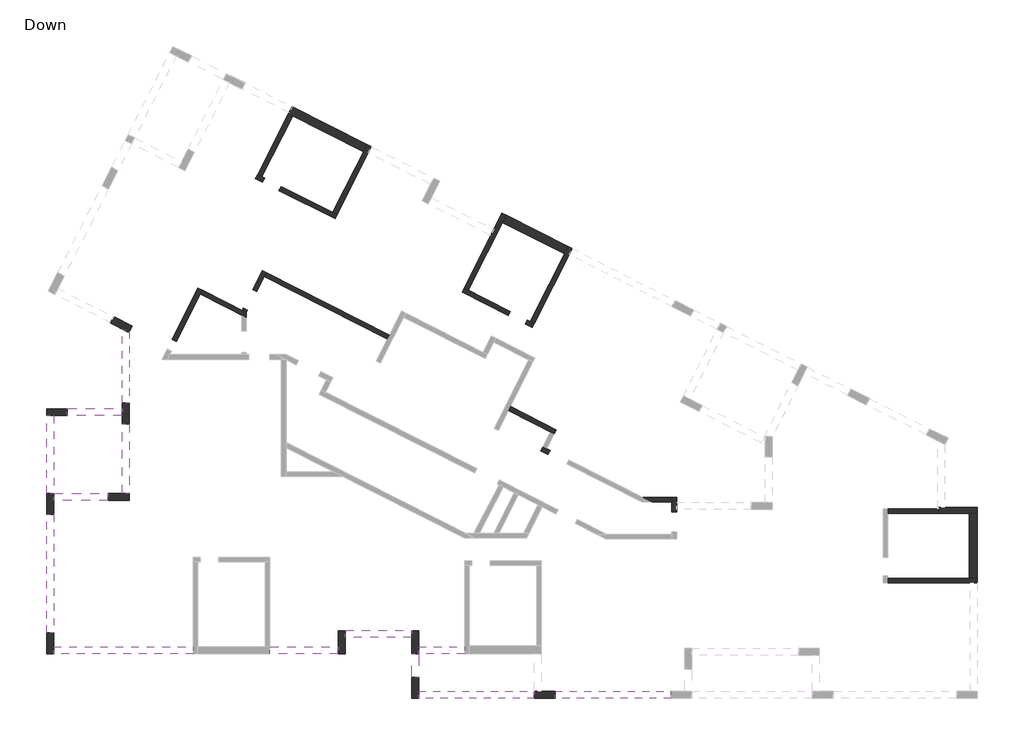
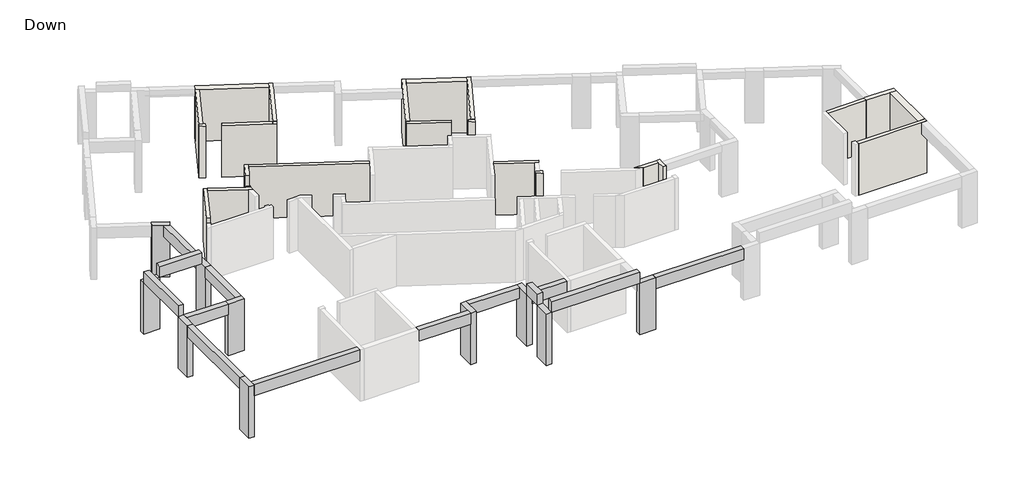
# One storey, part 2 of 3: 23 walls, 13 beams, 10 columns.
"""IFC4 building model written with IfcOpenShell, lengths in millimetres."""

from ifc_helpers import new_model, si_unit, frame, origin, origin_with_axes, place, context, project, spatial, polyline, outline, extrude, faceted_brep, element, save

model = new_model("IFC4")

# Units and contexts
model_context = context("Model", 3, world=origin())
ifc_project = project(units=[si_unit("LENGTHUNIT", "METRE", prefix="MILLI")], contexts=[model_context])

# Site, building, storey
site = spatial("IfcSite", under=ifc_project)
building = spatial("IfcBuilding", under=site)
storey = spatial("IfcBuildingStorey", under=building, Name="Down", Elevation=0.0)

# Beams
placement = place(None, origin())
element("IfcBeam", 1, ObjectType="Concrete Rectengular Beam : 30/65", at=placement, inside=storey, context=model_context, shape_type="SweptSolid", body=[
    extrude(outline(polyline([(-20357.3945771, -8406.9823068), (-20057.3945771, -8406.9823068), (-20057.3945771, -13520.1864188), (-20357.3945771, -13520.1864188), (-20357.3945771, -8406.9823068)])), frame((0.0, 0.0, 2430.0), z_axis=(0.0, 0.0, 1.0), x_axis=(1.0, 0.0, 0.0)), (0.0, 0.0, 1.0), 650.0),
])
element("IfcBeam", 2, ObjectType="Concrete Rectengular Beam : 30/65", at=placement, inside=storey, context=model_context, shape_type="Brep", body=[
    faceted_brep([(-17693.6398388, -7806.9823068, 3080.0), (-17693.6398388, -7506.9823068, 3080.0), (-20057.3945771, -7506.9823068, 3080.0), (-20057.3945771, -7806.9823068, 3080.0), (-20057.3945771, -7806.9823068, 2780.0), (-20057.3945771, -7806.9823068, 2430.0), (-17693.6398388, -7806.9823068, 2430.0), (-17693.6398388, -7806.9823068, 2780.0), (-17693.6398388, -7506.9823068, 2430.0), (-20057.3945771, -7506.9823068, 2430.0)], [[[0, 1, 2, 3]], [[0, 3, 4, 5, 6, 7]], [[8, 6, 5, 9]], [[1, 8, 9, 2]], [[1, 0, 7, 6, 8]], [[3, 2, 9, 5, 4]]]),
])
element("IfcBeam", 3, ObjectType="Concrete Rectengular Beam : 30/65", at=placement, inside=storey, context=model_context, shape_type="Brep", body=[
    faceted_brep([(-16793.6398388, -4507.7754014, 3080.0), (-17093.6398388, -4507.7754014, 3080.0), (-17093.6398388, -7506.9823068, 3080.0), (-16793.6398388, -7506.9823068, 3080.0), (-16793.6398388, -7506.9823068, 2780.0), (-16793.6398388, -7506.9823068, 2430.0), (-16793.6398388, -4507.7754014, 2430.0), (-16793.6398388, -4507.7754014, 2780.0), (-17093.6398388, -4507.7754014, 2430.0), (-17093.6398388, -7506.9823068, 2430.0)], [[[0, 1, 2, 3]], [[0, 3, 4, 5, 6, 7]], [[8, 6, 5, 9]], [[1, 8, 9, 2]], [[1, 0, 7, 6, 8]], [[3, 2, 9, 5, 4]]]),
])
element("IfcBeam", 4, ObjectType="Concrete Rectengular Beam : 30/65", at=placement, inside=storey, context=model_context, shape_type="Brep", body=[
    faceted_brep([(-17093.6398388, -3607.7754014, 3080.0), (-16793.6398388, -3607.7754014, 3080.0), (-16793.6398388, -532.9875537, 3080.0), (-16809.6695875, -564.4305223, 3080.0), (-17093.6398388, -419.6613746, 3080.0), (-16793.6398388, -3607.7754014, 2780.0), (-16793.6398388, -3607.7754014, 2430.0), (-16793.6398388, -532.9875537, 2430.0), (-16793.6398388, -532.9875537, 2780.0), (-17093.6398388, -3607.7754014, 2430.0), (-17093.6398388, -419.6613746, 2430.0), (-16809.6695875, -564.4305223, 2430.0)], [[[0, 1, 2, 3, 4]], [[2, 1, 5, 6, 7, 8]], [[6, 9, 10, 11, 7]], [[4, 10, 9, 0]], [[1, 0, 9, 6, 5]], [[3, 11, 10, 4]], [[11, 3, 2, 8, 7]]]),
])
element("IfcBeam", 5, ObjectType="Concrete Rectengular Beam : 30/65", at=placement, inside=storey, context=model_context, shape_type="Brep", body=[
    faceted_brep([(-20057.3945771, -14116.2328988, 3080.0), (-20057.3945771, -14416.2328988, 3080.0), (-14040.0148736, -14416.2328988, 3080.0), (-14040.0148736, -14116.2328988, 3080.0), (-20057.3945771, -14116.2328988, 2430.0), (-20057.3945771, -14116.2328988, 2780.0), (-14040.0148736, -14116.2328988, 2780.0), (-14040.0148736, -14116.2328988, 2430.0), (-20057.3945771, -14416.2328988, 2430.0), (-14040.0148736, -14416.2328988, 2430.0)], [[[0, 1, 2, 3]], [[4, 5, 0, 3, 6, 7]], [[8, 4, 7, 9]], [[1, 8, 9, 2]], [[1, 0, 5, 4, 8]], [[3, 2, 9, 7, 6]]]),
])
element("IfcBeam", 6, ObjectType="Concrete Rectengular Beam : 30/65", at=placement, inside=storey, context=model_context, shape_type="Brep", body=[
    faceted_brep([(-7799.9037617, -14416.2328988, 3080.0), (-7799.9037617, -14116.2328988, 3080.0), (-10738.2112055, -14116.2328988, 3080.0), (-10738.2112055, -14416.2328988, 3080.0), (-7799.9037617, -14416.2328988, 2430.0), (-10738.2112055, -14416.2328988, 2430.0), (-7799.9037617, -14116.2328988, 2430.0), (-10738.2112055, -14116.2328988, 2430.0), (-7799.9037617, -14116.2328988, 2780.0), (-10738.2112055, -14116.2328988, 2780.0)], [[[0, 1, 2, 3]], [[4, 0, 3, 5]], [[6, 4, 5, 7]], [[1, 8, 6, 7, 9, 2]], [[1, 0, 4, 6, 8]], [[3, 2, 9, 7, 5]]]),
])
element("IfcBeam", 7, ObjectType="Concrete Rectengular Beam : 30/65", at=placement, inside=storey, context=model_context, shape_type="Brep", body=[
    faceted_brep([(-7499.9037617, -13416.2328988, 3080.0), (-7499.9037617, -13716.2328988, 3080.0), (-4637.2823123, -13716.2328988, 3080.0), (-4637.2823123, -13416.2328988, 3080.0), (-7499.9037617, -13716.2328988, 2430.0), (-4637.2823123, -13716.2328988, 2430.0), (-7499.9037617, -13416.2328988, 2430.0), (-4637.2823123, -13416.2328988, 2430.0), (-4637.2823123, -13416.2328988, 2780.0), (-7499.9037617, -13416.2328988, 2780.0)], [[[0, 1, 2, 3]], [[1, 4, 5, 2]], [[4, 6, 7, 5]], [[0, 3, 8, 7, 6, 9]], [[1, 0, 9, 6, 4]], [[3, 2, 5, 7, 8]]]),
])
element("IfcBeam", 8, ObjectType="Concrete Rectengular Beam : 30/65", at=placement, inside=storey, context=model_context, shape_type="Brep", body=[
    faceted_brep([(-4337.2823123, -14116.2328988, 3080.0), (-4337.2823123, -14416.2328988, 3080.0), (-2356.7095864, -14416.2328988, 3080.0), (-2356.7095864, -14116.2328988, 3080.0), (-4337.2823123, -14416.2328988, 2430.0), (-2356.7095864, -14416.2328988, 2430.0), (-4337.2823123, -14116.2328988, 2430.0), (-2356.7095864, -14116.2328988, 2430.0), (-4337.2823123, -14116.2328988, 2780.0), (-2356.7095864, -14116.2328988, 2780.0)], [[[0, 1, 2, 3]], [[1, 4, 5, 2]], [[4, 6, 7, 5]], [[6, 8, 0, 3, 9, 7]], [[1, 0, 8, 6, 4]], [[3, 2, 5, 7, 9]]]),
])
element("IfcBeam", 9, ObjectType="Concrete Rectengular Beam : 30/65", at=placement, inside=storey, context=model_context, shape_type="SweptSolid", body=[
    extrude(outline(polyline([(1545.0940817, -16335.9823018), (1545.0940817, -16035.9823018), (6525.6343679, -16035.9823018), (6525.6343679, -16335.9823018), (1545.0940817, -16335.9823018)])), frame((0.0, 0.0, 2430.0), z_axis=(0.0, 0.0, 1.0), x_axis=(1.0, 0.0, 0.0)), (0.0, 0.0, 1.0), 650.0),
])
element("IfcBeam", 10, ObjectType="Concrete Rectengular Beam : 30/65", at=placement, inside=storey, context=model_context, shape_type="SweptSolid", body=[
    extrude(outline(polyline([(-20059.1333783, -7506.9823068), (-20359.1333783, -7506.9823068), (-20359.1333783, -4157.1728829), (-20059.1333783, -4157.1728829), (-20059.1333783, -7506.9823068)])), frame((0.0, 0.0, 3080.0), z_axis=(0.0, 0.0, 1.0), x_axis=(1.0, 0.0, 0.0)), (0.0, 0.0, 1.0), 650.0),
])
element("IfcBeam", 11, ObjectType="Concrete Rectengular Beam : 30/65", at=placement, inside=storey, context=model_context, shape_type="SweptSolid", body=[
    extrude(outline(polyline([(-17093.6398388, -3857.1728829), (-17093.6398388, -4157.1728829), (-19459.1333783, -4157.1728829), (-19459.1333783, -3857.1728829), (-17093.6398388, -3857.1728829)])), frame((0.0, 0.0, 3080.0), z_axis=(0.0, 0.0, 1.0), x_axis=(1.0, 0.0, 0.0)), (0.0, 0.0, 1.0), 650.0),
])
element("IfcBeam", 12, ObjectType="Concrete Rectengular Beam : 30/65", at=placement, inside=storey, context=model_context, shape_type="SweptSolid", body=[
    extrude(outline(polyline([(-4337.2823123, -15437.5523212), (-4637.2823123, -15437.5523212), (-4637.2823123, -14416.2328988), (-4337.2823123, -14416.2328988), (-4337.2823123, -15437.5523212)])), frame((0.0, 0.0, 3080.0), z_axis=(0.0, 0.0, 1.0), x_axis=(1.0, 0.0, 0.0)), (0.0, 0.0, 1.0), 650.0),
])
element("IfcBeam", 13, ObjectType="Concrete Rectengular Beam : 30/65", at=placement, inside=storey, context=model_context, shape_type="SweptSolid", body=[
    extrude(outline(polyline([(645.0940817, -16035.9823018), (645.0940817, -16335.9823018), (-4337.2823123, -16335.9823018), (-4337.2823123, -16035.9823018), (645.0940817, -16035.9823018)])), frame((0.0, 0.0, 3080.0), z_axis=(0.0, 0.0, 1.0), x_axis=(1.0, 0.0, 0.0)), (0.0, 0.0, 1.0), 650.0),
])

# Columns
element("IfcColumn", 14, ObjectType="Concrete Rectengular Column : 30/100", at=placement, inside=storey, context=model_context, shape_type="Brep", body=[
    faceted_brep([(-7499.9037617, -13416.2328988, 0.0), (-7499.9037617, -14416.2328988, 0.0), (-7799.9037617, -14416.2328988, 0.0), (-7799.9037617, -13416.2328988, 0.0), (-7499.9037617, -13416.2328988, 3080.0), (-7499.9037617, -14416.2328988, 3080.0), (-7799.9037617, -14416.2328988, 3080.0), (-7799.9037617, -14116.2328988, 3080.0), (-7799.9037617, -13416.2328988, 3080.0), (-7799.9037617, -13416.2328988, 2780.0)], [[[0, 1, 2, 3]], [[4, 5, 1, 0]], [[5, 6, 2, 1]], [[6, 7, 8, 9, 3, 2]], [[8, 4, 0, 3, 9]], [[4, 8, 7, 6, 5]]]),
])
element("IfcColumn", 15, ObjectType="Concrete Rectengular Column : 30/100", at=placement, inside=storey, context=model_context, shape_type="Brep", body=[
    faceted_brep([(-4337.2823123, -13416.2328988, 0.0), (-4337.2823123, -14416.2328988, 0.0), (-4637.2823123, -14416.2328988, 0.0), (-4637.2823123, -13416.2328988, 0.0), (-4337.2823123, -13416.2328988, 3080.0), (-4337.2823123, -14116.2328988, 3080.0), (-4337.2823123, -14416.2328988, 3080.0), (-4337.2823123, -13416.2328988, 2780.0), (-4637.2823123, -14416.2328988, 3080.0), (-4637.2823123, -13416.2328988, 3080.0)], [[[0, 1, 2, 3]], [[4, 5, 6, 1, 0, 7]], [[6, 8, 2, 1]], [[8, 9, 3, 2]], [[9, 4, 7, 0, 3]], [[4, 9, 8, 6, 5]]]),
])
element("IfcColumn", 16, ObjectType="Concrete Rectengular Column : 30/90", at=placement, inside=storey, context=model_context, shape_type="SweptSolid", body=[
    extrude(outline(polyline([(-20359.1333783, -3857.1728829), (-19459.1333783, -3857.1728829), (-19459.1333783, -4157.1728829), (-20359.1333783, -4157.1728829), (-20359.1333783, -3857.1728829)])), origin_with_axes(), (0.0, 0.0, 1.0), 3080.0),
])
element("IfcColumn", 17, ObjectType="Concrete Rectengular Column : 30/90", at=placement, inside=storey, context=model_context, shape_type="SweptSolid", body=[
    extrude(outline(polyline([(-17093.6398388, -4507.7754014), (-17093.6398388, -3607.7754014), (-16793.6398388, -3607.7754014), (-16793.6398388, -4507.7754014), (-17093.6398388, -4507.7754014)])), origin_with_axes(), (0.0, 0.0, 1.0), 3080.0),
])
element("IfcColumn", 18, ObjectType="Concrete Rectengular Column : 30/90", at=placement, inside=storey, context=model_context, shape_type="Brep", body=[
    faceted_brep([(-20357.3945771, -8406.9823068, 0.0), (-20357.3945771, -7506.9823068, 0.0), (-20057.3945771, -7506.9823068, 0.0), (-20057.3945771, -8406.9823068, 0.0), (-20357.3945771, -8406.9823068, 3080.0), (-20357.3945771, -7506.9823068, 3080.0), (-20057.3945771, -7506.9823068, 3080.0), (-20057.3945771, -7806.9823068, 3080.0), (-20057.3945771, -8406.9823068, 3080.0)], [[[0, 1, 2, 3]], [[4, 5, 1, 0]], [[5, 6, 2, 1]], [[6, 7, 8, 3, 2]], [[8, 4, 0, 3]], [[4, 8, 7, 6, 5]]]),
])
element("IfcColumn", 19, ObjectType="Concrete Rectengular Column : 30/90", at=placement, inside=storey, context=model_context, shape_type="Brep", body=[
    faceted_brep([(-16793.6398388, -7806.9823068, 0.0), (-17693.6398388, -7806.9823068, 0.0), (-17693.6398388, -7506.9823068, 0.0), (-16793.6398388, -7506.9823068, 0.0), (-16793.6398388, -7806.9823068, 3080.0), (-17693.6398388, -7806.9823068, 3080.0), (-16793.6398388, -7806.9823068, 2780.0), (-17693.6398388, -7506.9823068, 3080.0), (-16793.6398388, -7506.9823068, 3080.0)], [[[0, 1, 2, 3]], [[4, 5, 1, 0, 6]], [[5, 7, 2, 1]], [[7, 8, 3, 2]], [[8, 4, 6, 0, 3]], [[4, 8, 7, 5]]]),
])
element("IfcColumn", 20, ObjectType="Concrete Rectengular Column : 30/90", at=placement, inside=storey, context=model_context, shape_type="Brep", body=[
    faceted_brep([(-20057.3945771, -13520.1864188, 0.0), (-20057.3945771, -14420.1864188, 0.0), (-20357.3945771, -14420.1864188, 0.0), (-20357.3945771, -13520.1864188, 0.0), (-20057.3945771, -13520.1864188, 3080.0), (-20057.3945771, -14116.2328988, 3080.0), (-20057.3945771, -14420.1864188, 3080.0), (-20357.3945771, -14420.1864188, 3080.0), (-20357.3945771, -13520.1864188, 3080.0)], [[[0, 1, 2, 3]], [[4, 5, 6, 1, 0]], [[6, 7, 2, 1]], [[7, 8, 3, 2]], [[8, 4, 0, 3]], [[4, 8, 7, 6, 5]]]),
])
element("IfcColumn", 21, ObjectType="Concrete Rectengular Column : 30/90", at=placement, inside=storey, context=model_context, shape_type="SweptSolid", body=[
    extrude(outline(polyline([(-4337.2823123, -15437.5523212), (-4337.2823123, -16337.5523212), (-4637.2823123, -16337.5523212), (-4637.2823123, -15437.5523212), (-4337.2823123, -15437.5523212)])), origin_with_axes(), (0.0, 0.0, 1.0), 3080.0),
])
element("IfcColumn", 22, ObjectType="Concrete Rectengular Column : 30/90", at=placement, inside=storey, context=model_context, shape_type="Brep", body=[
    faceted_brep([(645.0940817, -16035.9823018, 0.0), (1545.0940817, -16035.9823018, 0.0), (1545.0940817, -16335.9823018, 0.0), (645.0940817, -16335.9823018, 0.0), (645.0940817, -16035.9823018, 3080.0), (945.0940817, -16035.9823018, 3080.0), (1545.0940817, -16035.9823018, 3080.0), (1545.0940817, -16335.9823018, 3080.0), (645.0940817, -16335.9823018, 3080.0)], [[[0, 1, 2, 3]], [[4, 5, 6, 1, 0]], [[6, 7, 2, 1]], [[7, 8, 3, 2]], [[8, 4, 0, 3]], [[4, 8, 7, 6, 5]]]),
])
element("IfcColumn", 23, ObjectType="Concrete Rectengular Column : 30/90", at=placement, inside=storey, context=model_context, shape_type="Brep", body=[
    faceted_brep([(-16809.6695875, -564.4305223, 0.0), (-17611.4851198, -155.6618196, 0.0), (-17475.2288855, 111.6100244, 0.0), (-16673.4133533, -297.1586783, 0.0), (-16809.6695875, -564.4305223, 3080.0), (-17611.4851198, -155.6618196, 3080.0), (-17611.4851198, -155.6618196, 2430.0), (-17475.2288855, 111.6100244, 3080.0), (-17475.2288855, 111.6100244, 2430.0), (-16673.4133533, -297.1586783, 3080.0), (-16793.6398388, -532.9875537, 3080.0)], [[[0, 1, 2, 3]], [[4, 5, 6, 1, 0]], [[5, 7, 8, 2, 1, 6]], [[7, 9, 3, 2, 8]], [[9, 10, 4, 0, 3]], [[4, 10, 9, 7, 5]]]),
])

# Walls
element("IfcWall", 24, ObjectType="20", at=placement, inside=storey, context=model_context, shape_type="Brep", body=[
    faceted_brep([(-14771.2670683, -962.4758986, 0.0), (-13751.0685018, 1077.9212344, 0.0), (-13661.6245504, 1256.8091372, 0.0), (-13661.6245504, 1256.8091372, 3080.0), (-13751.0685018, 1077.9212344, 3080.0), (-14771.2670683, -962.4758986, 3080.0), (-14771.2670683, -962.4758986, 2780.0), (-14950.1525065, -873.0331795, 0.0), (-14950.1525065, -873.0331795, 2780.0), (-14950.1525065, -873.0331795, 3080.0), (-13840.040473, 1347.1908875, 3080.0), (-13840.040473, 1347.1908875, 2780.0), (-13840.040473, 1347.1908875, 0.0)], [[[0, 1, 2, 3, 4, 5, 6]], [[7, 8, 9, 10, 11, 12]], [[2, 1, 0, 7, 12]], [[5, 4, 3, 10, 9]], [[0, 6, 5, 9, 8, 7]], [[3, 2, 12, 11, 10]]]),
])
element("IfcWall", 25, ObjectType="20", at=placement, inside=storey, context=model_context, shape_type="Brep", body=[
    faceted_brep([(-13751.0685018, 1077.9212344, 0.0), (-11960.5135249, 170.863779, 0.0), (-11760.5135249, 69.5479895, 0.0), (-11760.5135249, 69.5479895, 3080.0), (-11960.5135249, 170.863779, 3080.0), (-13751.0685018, 1077.9212344, 3080.0), (-13751.0685018, 1077.9212344, 2780.0), (-13661.6245504, 1256.8091372, 0.0), (-13661.6245504, 1256.8091372, 3080.0), (-11938.2560624, 383.7869427, 3080.0), (-11760.5135249, 293.7463151, 3080.0), (-11760.5135249, 293.7463151, 2780.0), (-11760.5135249, 293.7463151, 0.0), (-11938.2560624, 383.7869427, 0.0)], [[[0, 1, 2, 3, 4, 5, 6]], [[7, 8, 9, 10, 11, 12, 13]], [[2, 1, 0, 7, 13, 12]], [[5, 4, 3, 10, 9, 8]], [[0, 6, 5, 8, 7]], [[3, 2, 12, 11, 10]]]),
])
element("IfcWall", 26, ObjectType="20", at=placement, inside=storey, context=model_context, shape_type="Brep", body=[
    faceted_brep([(-11759.841961, 293.406115, 0.0), (-11713.8494576, 384.8014744, 0.0), (-11713.8494576, 384.8014744, 2780.0), (-11713.8494576, 384.8014744, 3080.0), (-11759.841961, 293.406115, 3080.0), (-11759.841961, 293.406115, 2780.0), (-11938.2560624, 383.7869427, 0.0), (-11938.2560624, 383.7869427, 2780.0), (-11938.2560624, 383.7869427, 3080.0), (-11892.5037799, 474.7049399, 3080.0), (-11892.5037799, 474.7049399, 2780.0), (-11892.5037799, 474.7049399, 0.0), (-11760.5135249, 293.7463151, 0.0), (-11760.5135249, 293.7463151, 3080.0)], [[[0, 1, 2, 3, 4, 5]], [[6, 7, 8, 9, 10, 11]], [[1, 0, 12, 6, 11]], [[3, 2, 1, 11, 10, 9]], [[4, 3, 9, 8, 13]], [[0, 5, 4, 13, 8, 7, 6, 12]]]),
])
element("IfcWall", 27, ObjectType="20", at=placement, inside=storey, context=model_context, shape_type="Brep", body=[
    faceted_brep([(-11309.677225, 1187.9642443, 0.0), (-10986.0255065, 1831.1183002, 0.0), (-10896.1212839, 2009.7741272, 0.0), (-10896.1212839, 2009.7741272, 3080.0), (-10986.0255065, 1831.1183002, 3080.0), (-11309.677225, 1187.9642443, 3080.0), (-11309.677225, 1187.9642443, 2780.0), (-11488.3315473, 1277.8677098, 0.0), (-11488.3315473, 1277.8677098, 2780.0), (-11488.3315473, 1277.8677098, 3080.0), (-11074.4066313, 2100.4108122, 3080.0), (-11074.4066313, 2100.4108122, 2780.0), (-11074.4066313, 2100.4108122, 0.0)], [[[0, 1, 2, 3, 4, 5, 6]], [[7, 8, 9, 10, 11, 12]], [[2, 1, 0, 7, 12]], [[5, 4, 3, 10, 9]], [[0, 6, 5, 9, 8, 7]], [[3, 2, 12, 11, 10]]]),
])
element("IfcWall", 28, ObjectType="20", at=placement, inside=storey, context=model_context, shape_type="Brep", body=[
    faceted_brep([(-10986.0255065, 1831.1183002, 0.0), (-5688.8111915, -861.8789214, 0.0), (-5688.8111915, -861.8789214, 2780.0), (-5688.8111915, -861.8789214, 3080.0), (-10986.0255065, 1831.1183002, 3080.0), (-10986.0255065, 1831.1183002, 2780.0), (-10896.1212839, 2009.7741272, 0.0), (-10896.1212839, 2009.7741272, 3080.0), (-5598.1752698, -683.5950755, 3080.0), (-5598.1752698, -683.5950755, 2780.0), (-5598.1752698, -683.5950755, 0.0)], [[[0, 1, 2, 3, 4, 5]], [[6, 7, 8, 9, 10]], [[1, 0, 6, 10]], [[4, 3, 8, 7]], [[0, 5, 4, 7, 6]], [[3, 2, 1, 10, 9, 8]]]),
])
element("IfcWall", 29, ObjectType="20", at=placement, inside=storey, context=model_context, shape_type="Brep", body=[
    faceted_brep([(-472.0818656, -3935.8417186, 0.0), (1327.1276693, -4852.636386, 0.0), (1505.3269714, -4943.4385782, 0.0), (1505.3269714, -4943.4385782, 3080.0), (1327.1276693, -4852.636386, 3080.0), (-472.0818656, -3935.8417186, 3080.0), (-472.0818656, -3935.8417186, 2780.0), (-382.0351871, -3757.2575237, 0.0), (-382.0351871, -3757.2575237, 2780.0), (-382.0351871, -3757.2575237, 3080.0), (1595.97634, -4765.1614866, 3080.0), (1595.97634, -4765.1614866, 2780.0), (1595.97634, -4765.1614866, 0.0)], [[[0, 1, 2, 3, 4, 5, 6]], [[7, 8, 9, 10, 11, 12]], [[2, 1, 0, 7, 12]], [[5, 4, 3, 10, 9]], [[0, 6, 5, 9, 8, 7]], [[3, 2, 12, 11, 10]]]),
])
element("IfcWall", 30, ObjectType="20", at=placement, inside=storey, context=model_context, shape_type="Brep", body=[
    faceted_brep([(910.387743, -5672.2249076, 0.0), (1232.0154262, -5834.8994051, 0.0), (1232.0154262, -5834.8994051, 2780.0), (1232.0154262, -5834.8994051, 3080.0), (910.387743, -5672.2249076, 3080.0), (910.387743, -5672.2249076, 2780.0), (1001.0372857, -5493.9474736, 0.0), (1001.0372857, -5493.9474736, 3080.0), (1179.5082357, -5584.2154251, 3080.0), (1322.2831712, -5656.4288636, 3080.0), (1322.2831712, -5656.4288636, 2780.0), (1322.2831712, -5656.4288636, 0.0), (1179.5082357, -5584.2154251, 0.0), (1275.5029536, -5748.919163, 3080.0)], [[[0, 1, 2, 3, 4, 5]], [[6, 7, 8, 9, 10, 11, 12]], [[1, 0, 6, 12, 11]], [[3, 2, 1, 11, 10, 9, 13]], [[4, 3, 13, 9, 8, 7]], [[0, 5, 4, 7, 6]]]),
])
element("IfcWall", 31, ObjectType="20", at=placement, inside=storey, context=model_context, shape_type="Brep", body=[
    faceted_brep([(5708.5555718, -7874.9401934, 0.0), (6570.8726693, -7874.9401934, 0.0), (6570.8726693, -7874.9401934, 2780.0), (6570.8726693, -7874.9401934, 3080.0), (5708.5555718, -7874.9401934, 3080.0), (5313.1307352, -7674.9401934, 0.0), (5313.1307352, -7674.9401934, 2780.0), (5313.1307352, -7674.9401934, 3080.0), (6570.8726693, -7674.9401934, 3080.0), (6570.8726693, -7674.9401934, 0.0)], [[[0, 1, 2, 3, 4]], [[5, 6, 7, 8, 9]], [[1, 0, 5, 9]], [[4, 3, 8, 7]], [[0, 4, 7, 6, 5]], [[3, 2, 1, 9, 8]]]),
])
element("IfcWall", 32, ObjectType="20", at=placement, inside=storey, context=model_context, shape_type="Brep", body=[
    faceted_brep([(6570.8726693, -7674.9401934, 0.0), (6570.8726693, -7874.9401934, 0.0), (6570.8726693, -8294.9401934, 0.0), (6570.8726693, -8294.9401934, 2780.0), (6570.8726693, -8294.9401934, 3080.0), (6570.8726693, -7874.9401934, 3080.0), (6570.8726693, -7674.9401934, 3080.0), (6770.8726693, -7674.9401934, 0.0), (6770.8726693, -7674.9401934, 2780.0), (6770.8726693, -7674.9401934, 3080.0), (6770.8726693, -7886.8724338, 3080.0), (6770.8726693, -8186.8724338, 3080.0), (6770.8726693, -8294.9401934, 3080.0), (6770.8726693, -8294.9401934, 2780.0), (6770.8726693, -8294.9401934, 0.0)], [[[0, 1, 2, 3, 4, 5, 6]], [[7, 8, 9, 10, 11, 12, 13, 14]], [[2, 1, 0, 7, 14]], [[4, 3, 2, 14, 13, 12]], [[6, 5, 4, 12, 11, 10, 9]], [[0, 6, 9, 8, 7]]]),
])
element("IfcWall", 33, ObjectType="20", at=placement, inside=storey, context=model_context, shape_type="Brep", body=[
    faceted_brep([(15870.9267875, -11368.4141282, 0.0), (19724.1024442, -11368.4141282, 0.0), (19724.1024442, -11368.4141282, 2430.0), (19724.1024442, -11368.4141282, 3080.0), (19424.1024442, -11368.4141282, 3080.0), (15870.9267875, -11368.4141282, 3080.0), (15870.9267875, -11168.4141282, 0.0), (15870.9267875, -11168.4141282, 2780.0), (15870.9267875, -11168.4141282, 3080.0), (19374.1024442, -11168.4141282, 3080.0), (19724.1024442, -11168.4141282, 3080.0), (19724.1024442, -11168.4141282, 0.0), (19374.1024442, -11168.4141282, 0.0)], [[[0, 1, 2, 3, 4, 5]], [[6, 7, 8, 9, 10, 11, 12]], [[1, 0, 6, 12, 11]], [[5, 4, 3, 10, 9, 8]], [[0, 5, 8, 7, 6]], [[3, 2, 1, 11, 10]]]),
])
element("IfcWall", 34, ObjectType="20", at=placement, inside=storey, context=model_context, shape_type="Brep", body=[
    faceted_brep([(15870.9267875, -8367.1461487, 0.0), (18025.5784419, -8367.1461487, 0.0), (18025.5784419, -8367.1461487, 3080.0), (15870.9267875, -8367.1461487, 3080.0), (15870.9267875, -8367.1461487, 2780.0), (15870.9267875, -8167.1461487, 0.0), (15870.9267875, -8167.1461487, 3080.0), (18024.1024442, -8167.1461487, 3080.0), (18025.5784419, -8167.1461487, 3080.0), (18025.5784419, -8167.1461487, 0.0)], [[[0, 1, 2, 3, 4]], [[5, 6, 7, 8, 9]], [[1, 0, 5, 9]], [[2, 1, 9, 8]], [[3, 2, 8, 7, 6]], [[0, 4, 3, 6, 5]]]),
])
element("IfcWall", 35, ObjectType="20", at=placement, inside=storey, context=model_context, shape_type="Brep", body=[
    faceted_brep([(2100.643933, 3136.6830555, 0.0), (1942.7646201, 2824.3144764, 0.0), (467.2492575, -95.0334036, 0.0), (467.2492575, -95.0334036, 2780.0), (467.2492575, -95.0334036, 3080.0), (1942.7646201, 2824.3144764, 3080.0), (2100.643933, 3136.6830555, 3080.0), (2279.1613083, 3046.5079542, 0.0), (2279.1613083, 3046.5079542, 2680.0), (2279.1613083, 3046.5079542, 3080.0), (2143.8361829, 2778.7634578, 3080.0), (645.7455836, -185.2501513, 3080.0), (645.7455836, -185.2501513, 2780.0), (645.7455836, -185.2501513, 0.0), (638.8365216, -181.7581293, 3080.0)], [[[0, 1, 2, 3, 4, 5, 6]], [[7, 8, 9, 10, 11, 12, 13]], [[2, 1, 0, 7, 13]], [[6, 5, 4, 14, 11, 10, 9]], [[4, 3, 2, 13, 12, 11, 14]], [[0, 6, 9, 8, 7]]]),
])
element("IfcWall", 36, ObjectType="20", at=placement, inside=storey, context=model_context, shape_type="Brep", body=[
    faceted_brep([(645.7455836, -185.2501513, 0.0), (467.2492575, -95.0334036, 0.0), (343.0939217, -32.2820245, 0.0), (343.0939217, -32.2820245, 3080.0), (467.2492575, -95.0334036, 3080.0), (645.7455836, -185.2501513, 3080.0), (555.5288358, -363.7464774, 0.0), (555.5288358, -363.7464774, 3080.0), (252.8771739, -210.7783506, 3080.0), (252.8771739, -210.7783506, 0.0)], [[[0, 1, 2, 3, 4, 5]], [[6, 7, 8, 9]], [[2, 1, 0, 6, 9]], [[3, 2, 9, 8]], [[5, 4, 3, 8, 7]], [[0, 5, 7, 6]]]),
])
element("IfcWall", 37, ObjectType="20", at=placement, inside=storey, context=model_context, shape_type="Brep", body=[
    faceted_brep([(-393.3542192, 339.9382762, 0.0), (-2196.5369883, 1251.3143734, 0.0), (-2375.0336984, 1341.5313152, 0.0), (-2375.0336984, 1341.5313152, 3080.0), (-2196.5369883, 1251.3143734, 3080.0), (-393.3542192, 339.9382762, 3080.0), (-393.3542192, 339.9382762, 2780.0), (-2464.8801865, 1162.8478502, 0.0), (-483.570967, 161.4419501, 0.0), (-483.570967, 161.4419501, 2780.0), (-483.570967, 161.4419501, 3080.0), (-2464.8801865, 1162.8478502, 3080.0), (-2464.8801865, 1162.8478502, 2780.0)], [[[0, 1, 2, 3, 4, 5, 6]], [[7, 8, 9, 10, 11, 12]], [[2, 1, 0, 8, 7]], [[5, 4, 3, 11, 10]], [[0, 6, 5, 10, 9, 8]], [[3, 2, 7, 12, 11]]]),
])
element("IfcWall", 38, ObjectType="20", at=placement, inside=storey, context=model_context, shape_type="Brep", body=[
    faceted_brep([(-2196.5369883, 1251.3143734, 0.0), (-727.390856, 4173.099378, 0.0), (-570.1595737, 4485.7952991, 0.0), (-570.1595737, 4485.7952991, 3080.0), (-727.390856, 4173.099378, 3080.0), (-2196.5369883, 1251.3143734, 3080.0), (-2196.5369883, 1251.3143734, 2780.0), (-2375.0336984, 1341.5313152, 0.0), (-2375.0336984, 1341.5313152, 3080.0), (-1236.2326264, 3606.3379414, 3080.0), (-748.6772466, 4575.9705507, 3080.0), (-748.6772466, 4575.9705507, 0.0)], [[[0, 1, 2, 3, 4, 5, 6]], [[7, 8, 9, 10, 11]], [[2, 1, 0, 7, 11]], [[5, 4, 3, 10, 9, 8]], [[0, 6, 5, 8, 7]], [[3, 2, 11, 10]]]),
])
element("IfcWall", 39, ObjectType="20", at=placement, inside=storey, context=model_context, shape_type="Brep", body=[
    faceted_brep([(-10350.4815757, 5543.7577579, 0.0), (-7938.3850799, 4337.70951, 0.0), (-7938.3850799, 4337.70951, 2780.0), (-7938.3850799, 4337.70951, 3080.0), (-10350.4815757, 5543.7577579, 3080.0), (-10261.0388566, 5722.6431961, 0.0), (-10261.0388566, 5722.6431961, 3080.0), (-8027.2639377, 4605.7557366, 3080.0), (-7848.3776081, 4516.3125718, 3080.0), (-7848.3776081, 4516.3125718, 0.0), (-8027.2639377, 4605.7557366, 0.0)], [[[0, 1, 2, 3, 4]], [[5, 6, 7, 8, 9, 10]], [[1, 0, 5, 10, 9]], [[4, 3, 8, 7, 6]], [[0, 4, 6, 5]], [[3, 2, 1, 9, 8]]]),
])
element("IfcWall", 40, ObjectType="20", at=placement, inside=storey, context=model_context, shape_type="Brep", body=[
    faceted_brep([(-7848.3776081, 4516.3125718, 0.0), (-6377.2019242, 7435.5866739, 0.0), (-6377.2019242, 7435.5866739, 2680.0), (-6377.2019242, 7435.5866739, 3080.0), (-6512.212519, 7167.6832976, 3080.0), (-7848.3776081, 4516.3125718, 3080.0), (-8027.2639377, 4605.7557366, 0.0), (-8027.2639377, 4605.7557366, 2780.0), (-8027.2639377, 4605.7557366, 3080.0), (-6713.2317343, 7213.2078736, 3080.0), (-6555.7193737, 7525.7618127, 3080.0), (-6555.7193737, 7525.7618127, 0.0), (-6713.2317343, 7213.2078736, 0.0)], [[[0, 1, 2, 3, 4, 5]], [[6, 7, 8, 9, 10, 11, 12]], [[1, 0, 6, 12, 11]], [[5, 4, 3, 10, 9, 8]], [[0, 5, 8, 7, 6]], [[3, 2, 1, 11, 10]]]),
])
element("IfcWall", 41, ObjectType="20", at=placement, inside=storey, context=model_context, shape_type="Brep", body=[
    faceted_brep([(-9944.2377987, 8845.2971792, 0.0), (-11274.3950333, 6229.3212844, 0.0), (-11274.3950333, 6229.3212844, 3080.0), (-9944.2377987, 8845.2971792, 3080.0), (-9765.7197974, 8755.1217618, 0.0), (-9765.7197974, 8755.1217618, 2780.0), (-9765.7197974, 8755.1217618, 3080.0), (-11095.5055118, 6139.8765236, 3080.0), (-11095.5055118, 6139.8765236, 2780.0), (-11095.5055118, 6139.8765236, 0.0)], [[[0, 1, 2, 3]], [[4, 5, 6, 7, 8, 9]], [[1, 0, 4, 9]], [[3, 2, 7, 6]], [[0, 3, 6, 5, 4]], [[2, 1, 9, 8, 7]]]),
])
element("IfcWall", 42, ObjectType="20", at=placement, inside=storey, context=model_context, shape_type="Brep", body=[
    faceted_brep([(-11365.0464378, 6051.0401889, 0.0), (-11060.9411929, 5898.9875664, 0.0), (-11060.9411929, 5898.9875664, 3080.0), (-11365.0464378, 6051.0401889, 3080.0), (-11274.3950333, 6229.3212844, 0.0), (-11274.3950333, 6229.3212844, 3080.0), (-11095.5055118, 6139.8765236, 3080.0), (-10971.4984738, 6077.8730046, 3080.0), (-10971.4984738, 6077.8730046, 2780.0), (-10971.4984738, 6077.8730046, 0.0), (-11095.5055118, 6139.8765236, 0.0)], [[[0, 1, 2, 3]], [[4, 5, 6, 7, 8, 9, 10]], [[1, 0, 4, 10, 9]], [[2, 1, 9, 8, 7]], [[3, 2, 7, 6, 5]], [[0, 3, 5, 4]]]),
])
element("IfcWall", 43, ObjectType="25", at=placement, inside=storey, context=model_context, shape_type="Brep", body=[
    faceted_brep([(18025.5784419, -8367.1461487, 0.0), (19374.1024442, -8367.1461487, 0.0), (19724.1024442, -8367.1461487, 0.0), (19724.1024442, -8367.1461487, 3080.0), (19374.1024442, -8367.1461487, 3080.0), (18025.5784419, -8367.1461487, 3080.0), (18025.5784419, -8117.1461487, 0.0), (18025.5784419, -8117.1461487, 3080.0), (19724.1024442, -8117.1461487, 3080.0), (19724.1024442, -8117.1461487, 0.0), (18025.5784419, -8167.1461487, 0.0), (18025.5784419, -8167.1461487, 3080.0)], [[[0, 1, 2, 3, 4, 5]], [[6, 7, 8, 9]], [[2, 1, 0, 10, 6, 9]], [[5, 4, 3, 8, 7, 11]], [[0, 5, 11, 7, 6, 10]], [[3, 2, 9, 8]]]),
])
element("IfcWall", 44, ObjectType="35", at=placement, inside=storey, context=model_context, shape_type="Brep", body=[
    faceted_brep([(19374.1024442, -8367.1461487, 0.0), (19374.1024442, -11168.4141282, 0.0), (19374.1024442, -11168.4141282, 2780.0), (19374.1024442, -11168.4141282, 3080.0), (19374.1024442, -8367.1461487, 3080.0), (19374.1024442, -8367.1461487, 2780.0), (19724.1024442, -8367.1461487, 0.0), (19724.1024442, -8367.1461487, 3080.0), (19724.1024442, -11168.4141282, 3080.0), (19724.1024442, -11168.4141282, 0.0)], [[[0, 1, 2, 3, 4, 5]], [[6, 7, 8, 9]], [[1, 0, 6, 9]], [[4, 3, 8, 7]], [[3, 2, 1, 9, 8]], [[0, 5, 4, 7, 6]]]),
])
element("IfcWall", 45, ObjectType="35", at=placement, inside=storey, context=model_context, shape_type="Brep", body=[
    faceted_brep([(-727.390856, 4173.099378, 0.0), (1942.7646201, 2824.3144764, 0.0), (1942.7646201, 2824.3144764, 3080.0), (-727.390856, 4173.099378, 3080.0), (-727.390856, 4173.099378, 2780.0), (-570.1595737, 4485.7952991, 0.0), (-570.1595737, 4485.7952991, 3080.0), (2100.643933, 3136.6830555, 3080.0), (2100.643933, 3136.6830555, 0.0)], [[[0, 1, 2, 3, 4]], [[5, 6, 7, 8]], [[1, 0, 5, 8]], [[3, 2, 7, 6]], [[0, 4, 3, 6, 5]], [[2, 1, 8, 7]]]),
])
element("IfcWall", 46, ObjectType="35", at=placement, inside=storey, context=model_context, shape_type="Brep", body=[
    faceted_brep([(-6555.7193737, 7525.7618127, 0.0), (-9785.6009014, 9157.2830771, 0.0), (-9785.6009014, 9157.2830771, 3080.0), (-6555.7193737, 7525.7618127, 3080.0), (-6713.2317343, 7213.2078736, 0.0), (-6713.2317343, 7213.2078736, 2780.0), (-6713.2317343, 7213.2078736, 3080.0), (-9765.7197974, 8755.1217618, 3080.0), (-9944.2377987, 8845.2971792, 3080.0), (-9944.2377987, 8845.2971792, 0.0), (-9765.7197974, 8755.1217618, 0.0)], [[[0, 1, 2, 3]], [[4, 5, 6, 7, 8, 9, 10]], [[1, 0, 4, 10, 9]], [[3, 2, 8, 7, 6]], [[0, 3, 6, 5, 4]], [[2, 1, 9, 8]]]),
])

save(model, "model.ifc")

# Revit data of these elements
# Type "Concrete Rectengular Beam : 30/65"
#   Length [instance default] = 152.4 cm
#   b = 30 cm
#   h = 65 cm
#   Structural Material [instance default] = Concrete
#   Assembly Code = ""
# Type "Concrete Rectengular Column : 30/100"
#   b = 30 cm
#   h = 100 cm
#   Structural Material [instance default] = Concrete
# Type "Concrete Rectengular Column : 30/90"
#   b = 30 cm
#   h = 90 cm
#   Structural Material [instance default] = Concrete
# Type "20"
#   Layers, outside or top first: 20 cm "Concrete" (function 1)
# Type "25"
#   Layers, outside or top first: 25 cm "Concrete" (function 1)
# Type "35"
#   Layers, outside or top first: 35 cm "Concrete" (function 1)
# Element 1 (IfcBeam, "Concrete Rectengular Beam : 30/65")
#   Comments = ""
#   Mark = "B17"
#   SOFiSTiK_AMG_Comments = ""
#   SOFiSTiK_AMG_Scheduled = yes
#   SOFiSTiK_AMG_Adjusted = yes
#   Structural Material = Concrete
#   Phase Created = New Construction
#   Materials on its faces: "Concrete"
# Element 2 (IfcBeam, "Concrete Rectengular Beam : 30/65")
#   Comments = ""
#   Mark = "B18"
#   SOFiSTiK_AMG_Comments = ""
#   SOFiSTiK_AMG_Scheduled = yes
#   SOFiSTiK_AMG_Adjusted = yes
#   Structural Material = Concrete
#   Phase Created = New Construction
#   Materials on its faces: "Concrete"
# Element 3 (IfcBeam, "Concrete Rectengular Beam : 30/65")
#   Comments = ""
#   Mark = "B19"
#   SOFiSTiK_AMG_Comments = ""
#   SOFiSTiK_AMG_Scheduled = yes
#   SOFiSTiK_AMG_Adjusted = yes
#   Structural Material = Concrete
#   Phase Created = New Construction
#   Materials on its faces: "Concrete"
# Element 4 (IfcBeam, "Concrete Rectengular Beam : 30/65")
#   Comments = ""
#   Mark = "B20"
#   SOFiSTiK_AMG_Comments = ""
#   SOFiSTiK_AMG_Scheduled = yes
#   SOFiSTiK_AMG_Adjusted = yes
#   Structural Material = Concrete
#   Phase Created = New Construction
#   Materials on its faces: "Concrete"
# Element 5 (IfcBeam, "Concrete Rectengular Beam : 30/65")
#   Comments = ""
#   Mark = "B26"
#   SOFiSTiK_AMG_Comments = ""
#   SOFiSTiK_AMG_Scheduled = yes
#   SOFiSTiK_AMG_Adjusted = yes
#   Structural Material = Concrete
#   Phase Created = New Construction
#   Materials on its faces: "Concrete"
# Element 6 (IfcBeam, "Concrete Rectengular Beam : 30/65")
#   Comments = ""
#   Mark = "B27"
#   SOFiSTiK_AMG_Comments = ""
#   SOFiSTiK_AMG_Scheduled = yes
#   SOFiSTiK_AMG_Adjusted = yes
#   Structural Material = Concrete
#   Phase Created = New Construction
#   Materials on its faces: "Concrete"
# Element 7 (IfcBeam, "Concrete Rectengular Beam : 30/65")
#   Comments = ""
#   Mark = "B28"
#   SOFiSTiK_AMG_Comments = ""
#   SOFiSTiK_AMG_Scheduled = yes
#   SOFiSTiK_AMG_Adjusted = yes
#   Structural Material = Concrete
#   Phase Created = New Construction
#   Materials on its faces: "Concrete"
# Element 8 (IfcBeam, "Concrete Rectengular Beam : 30/65")
#   Comments = ""
#   Mark = "B29"
#   SOFiSTiK_AMG_Comments = ""
#   SOFiSTiK_AMG_Scheduled = yes
#   SOFiSTiK_AMG_Adjusted = yes
#   Structural Material = Concrete
#   Phase Created = New Construction
#   Materials on its faces: "Concrete"
# Element 9 (IfcBeam, "Concrete Rectengular Beam : 30/65")
#   Comments = ""
#   Mark = "B31"
#   SOFiSTiK_AMG_Comments = ""
#   SOFiSTiK_AMG_Scheduled = yes
#   SOFiSTiK_AMG_Adjusted = yes
#   Structural Material = Concrete
#   Phase Created = New Construction
#   Materials on its faces: "Concrete"
# Element 10 (IfcBeam, "Concrete Rectengular Beam : 30/65")
#   Comments = ""
#   Mark = "B37"
#   SOFiSTiK_AMG_Comments = ""
#   SOFiSTiK_AMG_Scheduled = yes
#   SOFiSTiK_AMG_Adjusted = yes
#   Structural Material = Concrete
#   Phase Created = New Construction
#   Materials on its faces: "Concrete"
# Element 11 (IfcBeam, "Concrete Rectengular Beam : 30/65")
#   Comments = ""
#   Mark = "B38"
#   SOFiSTiK_AMG_Comments = ""
#   SOFiSTiK_AMG_Scheduled = yes
#   SOFiSTiK_AMG_Adjusted = yes
#   Structural Material = Concrete
#   Phase Created = New Construction
#   Materials on its faces: "Concrete"
# Element 12 (IfcBeam, "Concrete Rectengular Beam : 30/65")
#   Comments = ""
#   Mark = "B39"
#   SOFiSTiK_AMG_Comments = ""
#   SOFiSTiK_AMG_Scheduled = yes
#   SOFiSTiK_AMG_Adjusted = yes
#   Structural Material = Concrete
#   Phase Created = New Construction
#   Materials on its faces: "Concrete"
# Element 13 (IfcBeam, "Concrete Rectengular Beam : 30/65")
#   Comments = ""
#   Mark = "B40"
#   SOFiSTiK_AMG_Comments = ""
#   SOFiSTiK_AMG_Scheduled = yes
#   SOFiSTiK_AMG_Adjusted = yes
#   Structural Material = Concrete
#   Phase Created = New Construction
#   Materials on its faces: "Concrete"
# Element 14 (IfcColumn, "Concrete Rectengular Column : 30/100")
#   Comments = ""
#   Mark = "C1"
#   SOFiSTiK_AMG_Comments = ""
#   SOFiSTiK_AMG_Scheduled = yes
#   SOFiSTiK_AMG_Adjusted = yes
#   Structural Material = Concrete
#   Phase Created = New Construction
#   Materials on its faces: "Concrete"
# Element 15 (IfcColumn, "Concrete Rectengular Column : 30/100")
#   Comments = ""
#   Mark = "C2"
#   SOFiSTiK_AMG_Comments = ""
#   SOFiSTiK_AMG_Scheduled = yes
#   SOFiSTiK_AMG_Adjusted = yes
#   Structural Material = Concrete
#   Phase Created = New Construction
#   Materials on its faces: "Concrete"
# Element 16 (IfcColumn, "Concrete Rectengular Column : 30/90")
#   Comments = ""
#   Mark = "C6"
#   SOFiSTiK_AMG_Comments = ""
#   SOFiSTiK_AMG_Scheduled = yes
#   SOFiSTiK_AMG_Adjusted = yes
#   Structural Material = Concrete
#   Phase Created = New Construction
#   Materials on its faces: "Concrete"
# Element 17 (IfcColumn, "Concrete Rectengular Column : 30/90")
#   Comments = ""
#   Mark = "C7"
#   SOFiSTiK_AMG_Comments = ""
#   SOFiSTiK_AMG_Scheduled = yes
#   SOFiSTiK_AMG_Adjusted = yes
#   Structural Material = Concrete
#   Phase Created = New Construction
#   Materials on its faces: "Concrete"
# Element 18 (IfcColumn, "Concrete Rectengular Column : 30/90")
#   Comments = ""
#   Mark = "C8"
#   SOFiSTiK_AMG_Comments = ""
#   SOFiSTiK_AMG_Scheduled = yes
#   SOFiSTiK_AMG_Adjusted = yes
#   Structural Material = Concrete
#   Phase Created = New Construction
#   Materials on its faces: "Concrete"
# Element 19 (IfcColumn, "Concrete Rectengular Column : 30/90")
#   Comments = ""
#   Mark = "C9"
#   SOFiSTiK_AMG_Comments = ""
#   SOFiSTiK_AMG_Scheduled = yes
#   SOFiSTiK_AMG_Adjusted = yes
#   Structural Material = Concrete
#   Phase Created = New Construction
#   Materials on its faces: "Concrete"
# Element 20 (IfcColumn, "Concrete Rectengular Column : 30/90")
#   Comments = ""
#   Mark = "C10"
#   SOFiSTiK_AMG_Comments = ""
#   SOFiSTiK_AMG_Scheduled = yes
#   SOFiSTiK_AMG_Adjusted = yes
#   Structural Material = Concrete
#   Phase Created = New Construction
#   Materials on its faces: "Concrete"
# Element 21 (IfcColumn, "Concrete Rectengular Column : 30/90")
#   Comments = ""
#   Mark = "C11"
#   SOFiSTiK_AMG_Comments = ""
#   SOFiSTiK_AMG_Scheduled = yes
#   SOFiSTiK_AMG_Adjusted = yes
#   Structural Material = Concrete
#   Phase Created = New Construction
#   Materials on its faces: "Concrete"
# Element 22 (IfcColumn, "Concrete Rectengular Column : 30/90")
#   Comments = ""
#   Mark = "C12"
#   SOFiSTiK_AMG_Comments = ""
#   SOFiSTiK_AMG_Scheduled = yes
#   SOFiSTiK_AMG_Adjusted = yes
#   Structural Material = Concrete
#   Phase Created = New Construction
#   Materials on its faces: "Concrete"
# Element 23 (IfcColumn, "Concrete Rectengular Column : 30/90")
#   Comments = ""
#   Mark = "C27"
#   SOFiSTiK_AMG_Comments = ""
#   SOFiSTiK_AMG_Scheduled = yes
#   SOFiSTiK_AMG_Adjusted = yes
#   Structural Material = Concrete
#   Phase Created = New Construction
#   Materials on its faces: "Concrete"
# Element 24 (IfcWall, "20")
#   Comments = ""
#   Mark = "W5"
#   SOFiSTiK_AMG_Comments = ""
#   Top Offset = 0 cm
#   Base Offset = 0 cm
#   wall height = 308 cm
#   SOFiSTiK_AMG_Scheduled = yes
#   SOFiSTiK_AMG_Adjusted = yes
#   Phase Created = New Construction
#   Base Constraint = Down
#   Top Constraint = Typical Floor
#   Materials on its faces: "Concrete"
# Element 25 (IfcWall, "20")
#   Comments = ""
#   Mark = "W6"
#   SOFiSTiK_AMG_Comments = ""
#   Top Offset = 0 cm
#   Base Offset = 0 cm
#   wall height = 308 cm
#   SOFiSTiK_AMG_Scheduled = yes
#   SOFiSTiK_AMG_Adjusted = yes
#   Phase Created = New Construction
#   Base Constraint = Down
#   Top Constraint = Typical Floor
#   Materials on its faces: "Concrete"
# Element 26 (IfcWall, "20")
#   Comments = ""
#   Mark = "W9"
#   SOFiSTiK_AMG_Comments = "Too Short /"
#   Top Offset = 0 cm
#   Base Offset = 0 cm
#   wall height = 308 cm
#   SOFiSTiK_AMG_Scheduled = yes
#   SOFiSTiK_AMG_Adjusted = yes
#   Phase Created = New Construction
#   Base Constraint = Down
#   Top Constraint = Typical Floor
#   Materials on its faces: "Concrete"
# Element 27 (IfcWall, "20")
#   Comments = ""
#   Mark = "W10"
#   SOFiSTiK_AMG_Comments = ""
#   Top Offset = 0 cm
#   Base Offset = 0 cm
#   wall height = 308 cm
#   SOFiSTiK_AMG_Scheduled = yes
#   SOFiSTiK_AMG_Adjusted = yes
#   Phase Created = New Construction
#   Base Constraint = Down
#   Top Constraint = Typical Floor
#   Materials on its faces: "Concrete"
# Element 28 (IfcWall, "20")
#   Comments = ""
#   Mark = "W11"
#   SOFiSTiK_AMG_Comments = ""
#   Top Offset = 0 cm
#   Base Offset = 0 cm
#   wall height = 308 cm
#   SOFiSTiK_AMG_Scheduled = yes
#   SOFiSTiK_AMG_Adjusted = yes
#   Phase Created = New Construction
#   Base Constraint = Down
#   Top Constraint = Typical Floor
#   Materials on its faces: "Concrete"
# Element 29 (IfcWall, "20")
#   Comments = ""
#   Mark = "W17"
#   SOFiSTiK_AMG_Comments = ""
#   Top Offset = 0 cm
#   Base Offset = 0 cm
#   wall height = 308 cm
#   SOFiSTiK_AMG_Scheduled = yes
#   SOFiSTiK_AMG_Adjusted = yes
#   Phase Created = New Construction
#   Base Constraint = Down
#   Top Constraint = Typical Floor
#   Materials on its faces: "Concrete"
# Element 30 (IfcWall, "20")
#   Comments = ""
#   Mark = "W19"
#   SOFiSTiK_AMG_Comments = ""
#   Top Offset = 0 cm
#   Base Offset = 0 cm
#   wall height = 308 cm
#   SOFiSTiK_AMG_Scheduled = yes
#   SOFiSTiK_AMG_Adjusted = yes
#   Phase Created = New Construction
#   Base Constraint = Down
#   Top Constraint = Typical Floor
#   Materials on its faces: "Concrete"
# Element 31 (IfcWall, "20")
#   Comments = ""
#   Mark = "W21"
#   SOFiSTiK_AMG_Comments = ""
#   Top Offset = 0 cm
#   Base Offset = 0 cm
#   wall height = 308 cm
#   SOFiSTiK_AMG_Scheduled = yes
#   SOFiSTiK_AMG_Adjusted = yes
#   Phase Created = New Construction
#   Base Constraint = Down
#   Top Constraint = Typical Floor
#   Materials on its faces: "Concrete"
# Element 32 (IfcWall, "20")
#   Comments = ""
#   Mark = "W22"
#   SOFiSTiK_AMG_Comments = ""
#   Top Offset = 0 cm
#   Base Offset = 0 cm
#   wall height = 308 cm
#   SOFiSTiK_AMG_Scheduled = yes
#   SOFiSTiK_AMG_Adjusted = yes
#   Phase Created = New Construction
#   Base Constraint = Down
#   Top Constraint = Typical Floor
#   Materials on its faces: "Concrete"
# Element 33 (IfcWall, "20")
#   Comments = ""
#   Mark = "W40"
#   SOFiSTiK_AMG_Comments = ""
#   Top Offset = 0 cm
#   Base Offset = 0 cm
#   wall height = 308 cm
#   SOFiSTiK_AMG_Scheduled = yes
#   SOFiSTiK_AMG_Adjusted = yes
#   Phase Created = New Construction
#   Base Constraint = Down
#   Top Constraint = Typical Floor
#   Materials on its faces: "Concrete"
# Element 34 (IfcWall, "20")
#   Comments = ""
#   Mark = "W42"
#   SOFiSTiK_AMG_Comments = ""
#   Top Offset = 0 cm
#   Base Offset = 0 cm
#   wall height = 308 cm
#   SOFiSTiK_AMG_Scheduled = yes
#   SOFiSTiK_AMG_Adjusted = yes
#   Phase Created = New Construction
#   Base Constraint = Down
#   Top Constraint = Typical Floor
#   Materials on its faces: "Concrete"
# Element 35 (IfcWall, "20")
#   Comments = ""
#   Mark = "W43"
#   SOFiSTiK_AMG_Comments = ""
#   Top Offset = 0 cm
#   Base Offset = 0 cm
#   wall height = 308 cm
#   SOFiSTiK_AMG_Scheduled = yes
#   SOFiSTiK_AMG_Adjusted = yes
#   Phase Created = New Construction
#   Base Constraint = Down
#   Top Constraint = Typical Floor
#   Materials on its faces: "Concrete"
# Element 36 (IfcWall, "20")
#   Comments = ""
#   Mark = "W44"
#   SOFiSTiK_AMG_Comments = ""
#   Top Offset = 0 cm
#   Base Offset = 0 cm
#   wall height = 308 cm
#   SOFiSTiK_AMG_Scheduled = yes
#   SOFiSTiK_AMG_Adjusted = yes
#   Phase Created = New Construction
#   Base Constraint = Down
#   Top Constraint = Typical Floor
#   Materials on its faces: "Concrete"
# Element 37 (IfcWall, "20")
#   Comments = ""
#   Mark = "W45"
#   SOFiSTiK_AMG_Comments = ""
#   Top Offset = 0 cm
#   Base Offset = 0 cm
#   wall height = 308 cm
#   SOFiSTiK_AMG_Scheduled = yes
#   SOFiSTiK_AMG_Adjusted = yes
#   Phase Created = New Construction
#   Base Constraint = Down
#   Top Constraint = Typical Floor
#   Materials on its faces: "Concrete"
# Element 38 (IfcWall, "20")
#   Comments = ""
#   Mark = "W46"
#   SOFiSTiK_AMG_Comments = ""
#   Top Offset = 0 cm
#   Base Offset = 0 cm
#   wall height = 308 cm
#   SOFiSTiK_AMG_Scheduled = yes
#   SOFiSTiK_AMG_Adjusted = yes
#   Phase Created = New Construction
#   Base Constraint = Down
#   Top Constraint = Typical Floor
#   Materials on its faces: "Concrete"
# Element 39 (IfcWall, "20")
#   Comments = ""
#   Mark = "W47"
#   SOFiSTiK_AMG_Comments = ""
#   Top Offset = 0 cm
#   Base Offset = 0 cm
#   wall height = 308 cm
#   SOFiSTiK_AMG_Scheduled = yes
#   SOFiSTiK_AMG_Adjusted = yes
#   Phase Created = New Construction
#   Base Constraint = Down
#   Top Constraint = Typical Floor
#   Materials on its faces: "Concrete"
# Element 40 (IfcWall, "20")
#   Comments = ""
#   Mark = "W48"
#   SOFiSTiK_AMG_Comments = ""
#   Top Offset = 0 cm
#   Base Offset = 0 cm
#   wall height = 308 cm
#   SOFiSTiK_AMG_Scheduled = yes
#   SOFiSTiK_AMG_Adjusted = yes
#   Phase Created = New Construction
#   Base Constraint = Down
#   Top Constraint = Typical Floor
#   Materials on its faces: "Concrete"
# Element 41 (IfcWall, "20")
#   Comments = ""
#   Mark = "W49"
#   SOFiSTiK_AMG_Comments = ""
#   Top Offset = 0 cm
#   Base Offset = 0 cm
#   wall height = 308 cm
#   SOFiSTiK_AMG_Scheduled = yes
#   SOFiSTiK_AMG_Adjusted = yes
#   Phase Created = New Construction
#   Base Constraint = Down
#   Top Constraint = Typical Floor
#   Materials on its faces: "Concrete"
# Element 42 (IfcWall, "20")
#   Comments = ""
#   Mark = "W50"
#   SOFiSTiK_AMG_Comments = ""
#   Top Offset = 0 cm
#   Base Offset = 0 cm
#   wall height = 308 cm
#   SOFiSTiK_AMG_Scheduled = yes
#   SOFiSTiK_AMG_Adjusted = yes
#   Phase Created = New Construction
#   Base Constraint = Down
#   Top Constraint = Typical Floor
#   Materials on its faces: "Concrete"
# Element 43 (IfcWall, "25")
#   Comments = ""
#   Mark = "W62"
#   SOFiSTiK_AMG_Comments = ""
#   Top Offset = 0 cm
#   Base Offset = 0 cm
#   wall height = 308 cm
#   SOFiSTiK_AMG_Scheduled = yes
#   SOFiSTiK_AMG_Adjusted = yes
#   Phase Created = New Construction
#   Base Constraint = Down
#   Top Constraint = Typical Floor
#   Materials on its faces: "Concrete"
# Element 44 (IfcWall, "35")
#   Comments = ""
#   Mark = "W59"
#   SOFiSTiK_AMG_Comments = ""
#   Top Offset = 0 cm
#   Base Offset = 0 cm
#   wall height = 308 cm
#   SOFiSTiK_AMG_Scheduled = yes
#   SOFiSTiK_AMG_Adjusted = yes
#   Phase Created = New Construction
#   Base Constraint = Down
#   Top Constraint = Typical Floor
#   Materials on its faces: "Concrete"
# Element 45 (IfcWall, "35")
#   Comments = ""
#   Mark = "W60"
#   SOFiSTiK_AMG_Comments = ""
#   Top Offset = 0 cm
#   Base Offset = 0 cm
#   wall height = 308 cm
#   SOFiSTiK_AMG_Scheduled = yes
#   SOFiSTiK_AMG_Adjusted = yes
#   Phase Created = New Construction
#   Base Constraint = Down
#   Top Constraint = Typical Floor
#   Materials on its faces: "Concrete"
# Element 46 (IfcWall, "35")
#   Comments = ""
#   Mark = "W61"
#   SOFiSTiK_AMG_Comments = ""
#   Top Offset = 0 cm
#   Base Offset = 0 cm
#   wall height = 308 cm
#   SOFiSTiK_AMG_Scheduled = yes
#   SOFiSTiK_AMG_Adjusted = yes
#   Phase Created = New Construction
#   Base Constraint = Down
#   Top Constraint = Typical Floor
#   Materials on its faces: "Concrete"
# Materials
#   "Concrete": class "Concrete", colour RGB 192 192 192, transparency 0, Keynote = "01000", Description = "Cast-in-place concrete", Cost = 0
